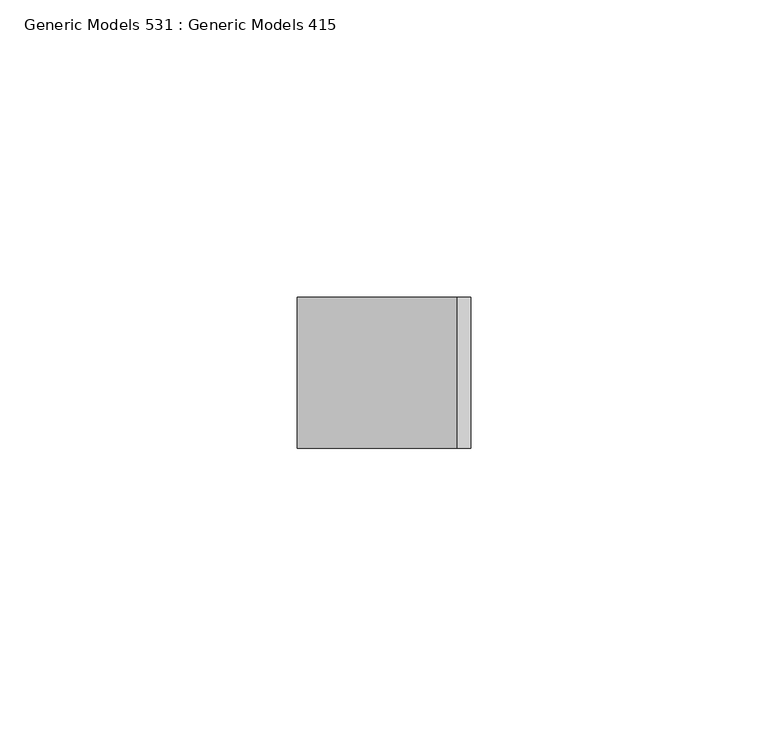
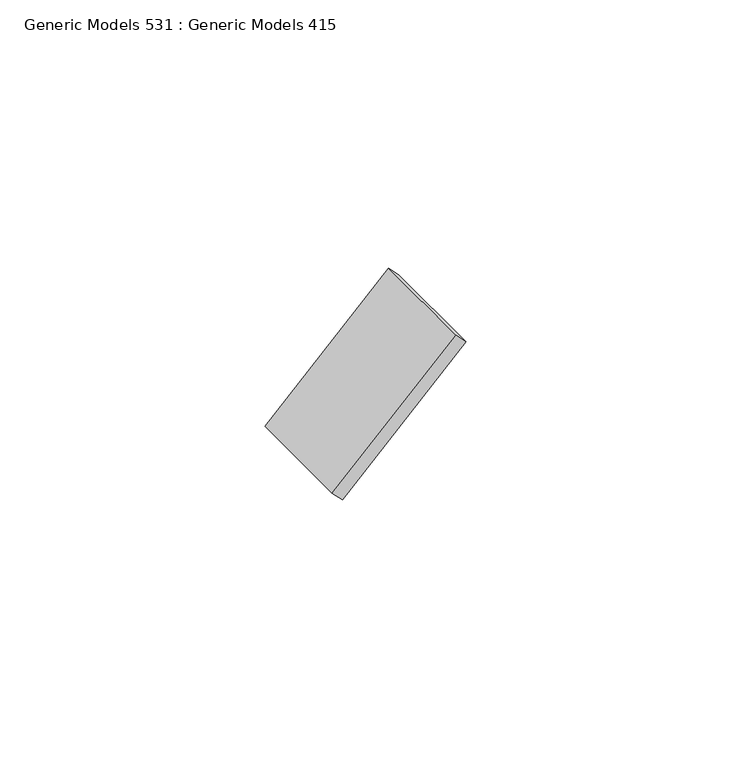
"""IFC4 building model written with IfcOpenShell, lengths in millimetres: proxy geometry, Generic Models 531 : Generic Models 415."""

from ifc_helpers import new_model, si_unit, frame, origin, place, context, project, spatial, polyline, outline, extrude, source, transform, mapped, element, save


def generic_models_531_generic_models_415_9d641313(model_context):
    return source(origin(), model_context, "Body", "SweptSolid", [
        extrude(outline(polyline([(0.0, -3.175), (0.0, 0.0), (25.4, 0.0), (25.4, -3.175), (0.0, -3.175)])), frame((7848.0411784, 4501.3863946, 125321.3849742), z_axis=(0.7071067811867181, 0.0, 0.707106781186377), x_axis=(0.0, -1.0, 0.0)), (0.0, 0.0, 1.0), 38.1),
    ])


if __name__ == "__main__":
    model = new_model("IFC4")
    model_context = context("Model", 3, world=origin())
    ifc_project = project(units=[si_unit("LENGTHUNIT", "METRE", prefix="MILLI")], contexts=[model_context])
    site = spatial("IfcSite", under=ifc_project)
    building = spatial("IfcBuilding", under=site)
    placement = place(None, origin())
    generic_models_531_generic_models_415_shape = generic_models_531_generic_models_415_9d641313(model_context)
    element("IfcBuildingElementProxy", 1, Name="Generic Models 531 : Generic Models 415", ObjectType="Generic Models 531 : Generic Models 415", at=placement, inside=building, context=model_context, shape_type="MappedRepresentation", body=[
        mapped(generic_models_531_generic_models_415_shape, transform((0.0, 0.0, 0.0), x_axis=(1.0, 0.0, 0.0), y_axis=(0.0, 1.0, 0.0), z_axis=(0.0, 0.0, 1.0))),
    ])
    save(model, "model.ifc")

# Revit data of these elements
# Element 1 (IfcBuildingElementProxy, "Generic Models 531 : Generic Models 415")
#   Materials on its faces: "_WELDED STEEL TABS FOR LOUVER ATTACHMENT"
# Materials
#   "_WELDED STEEL TABS FOR LOUVER ATTACHMENT": class "Metal", colour RGB 199 199 199, transparency 0, Description = "Structural steel 50ksi", Cost = 0
